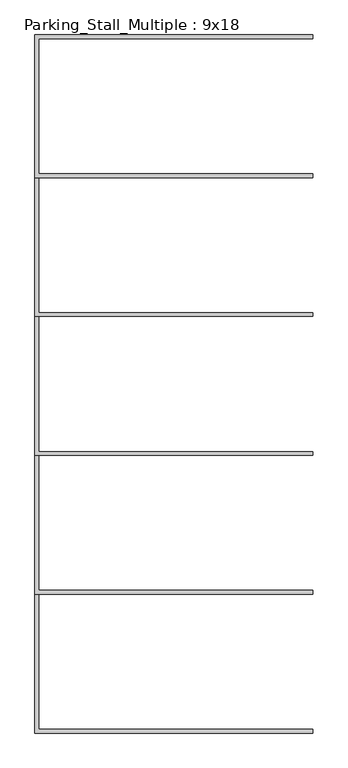
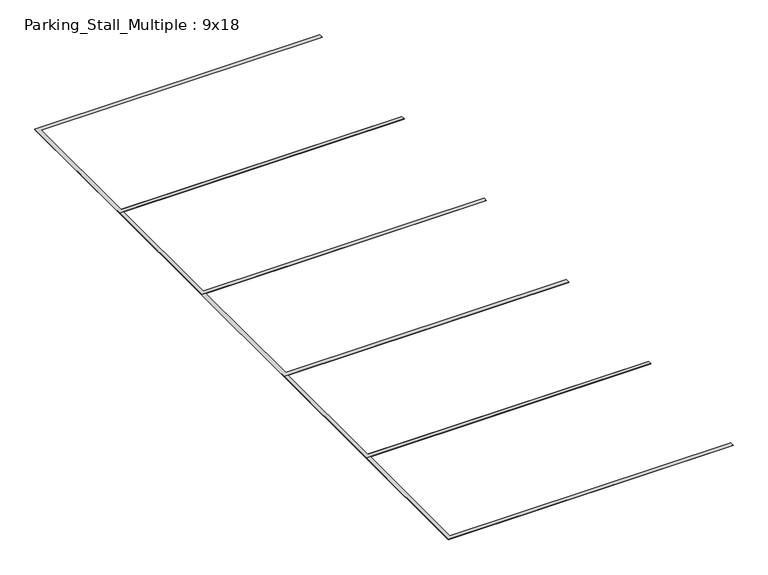
"""IFC4 building model written with IfcOpenShell, lengths in millimetres: proxy geometry, Parking_Stall_Multiple : 9x18."""

from ifc_helpers import new_model, si_unit, origin, origin_with_axes, place, context, project, spatial, polyline, outline, extrude, source, transform, mapped, element, save


def parking_stall_multiple_9x18_ed2115c2(model_context):
    return source(origin(), model_context, "Body", "SweptSolid", [
        extrude(outline(polyline([(5486.4, 10972.8), (0.0, 10972.8), (0.0, 13792.2), (5486.4, 13792.2), (5486.4, 13716.0), (76.2, 13716.0), (76.2, 11049.0), (5486.4, 11049.0), (5486.4, 10972.8)])), origin_with_axes(), (0.0, 0.0, 1.0), 6.35),
        extrude(outline(polyline([(5486.4, 8229.6), (0.0, 8229.6), (0.0, 11049.0), (5486.4, 11049.0), (5486.4, 10972.8), (76.2, 10972.8), (76.2, 8305.8), (5486.4, 8305.8), (5486.4, 8229.6)])), origin_with_axes(), (0.0, 0.0, 1.0), 6.35),
        extrude(outline(polyline([(5486.4, 5486.4), (0.0, 5486.4), (0.0, 8305.8), (5486.4, 8305.8), (5486.4, 8229.6), (76.2, 8229.6), (76.2, 5562.6), (5486.4, 5562.6), (5486.4, 5486.4)])), origin_with_axes(), (0.0, 0.0, 1.0), 6.35),
        extrude(outline(polyline([(5486.4, 2743.2), (0.0, 2743.2), (0.0, 5562.6), (5486.4, 5562.6), (5486.4, 5486.4), (76.2, 5486.4), (76.2, 2819.4), (5486.4, 2819.4), (5486.4, 2743.2)])), origin_with_axes(), (0.0, 0.0, 1.0), 6.35),
        extrude(outline(polyline([(5486.4, 0.0), (0.0, 0.0), (0.0, 2819.4), (5486.4, 2819.4), (5486.4, 2743.2), (76.2, 2743.2), (76.2, 76.2), (5486.4, 76.2), (5486.4, 0.0)])), origin_with_axes(), (0.0, 0.0, 1.0), 6.35),
    ])


if __name__ == "__main__":
    model = new_model("IFC4")
    model_context = context("Model", 3, world=origin())
    ifc_project = project(units=[si_unit("LENGTHUNIT", "METRE", prefix="MILLI")], contexts=[model_context])
    site = spatial("IfcSite", under=ifc_project)
    building = spatial("IfcBuilding", under=site)
    placement = place(None, origin())
    parking_stall_multiple_9x18_shape = parking_stall_multiple_9x18_ed2115c2(model_context)
    element("IfcBuildingElementProxy", 1, Name="Parking_Stall_Multiple : 9x18", ObjectType="Parking_Stall_Multiple : 9x18", at=placement, inside=building, context=model_context, shape_type="MappedRepresentation", body=[
        mapped(parking_stall_multiple_9x18_shape, transform((0.0, 0.0, 0.0), x_axis=(1.0, 0.0, 0.0), y_axis=(0.0, 1.0, 0.0), z_axis=(0.0, 0.0, 1.0))),
    ])
    save(model, "model.ifc")

# Revit data of these elements
# Type "Parking_Stall_Multiple : 9x18"
#   Parking_Width_M = 9' - 0"
#   Parking_Run_Length [instance default] = 65' - 0"
#   Parking_Line_Width = 0' - 3"
#   Parking_Length_M = 18' - 0"
#   Single_Parking_Visibility [instance default] = no
#   Parking_ADA_Symbol = no
#   ParkingUnitsArray [instance default] = 7
#   ParkingUnits [instance default] = 7
#   Multiple_Parking_Visibility [instance default] = yes
#   Parking_Line_Material = none
# Element 1 (IfcBuildingElementProxy, "Parking_Stall_Multiple : 9x18")
#   Parking_Run_Length = 45' - 4.43699"
#   ParkingUnitsArray = 5
#   ParkingUnits = 5
